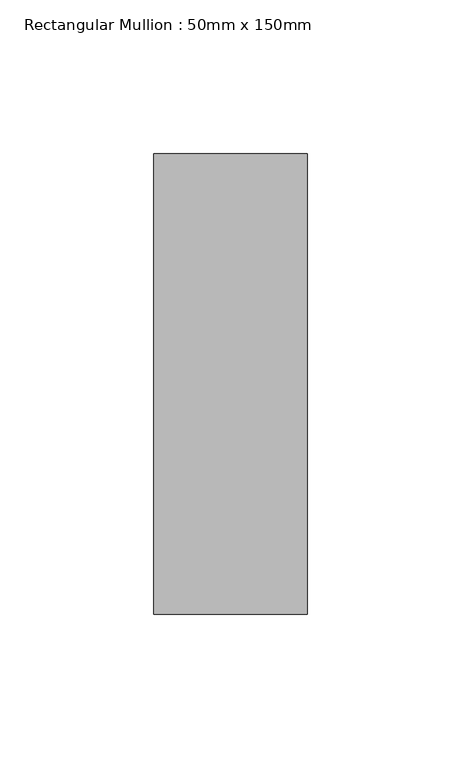
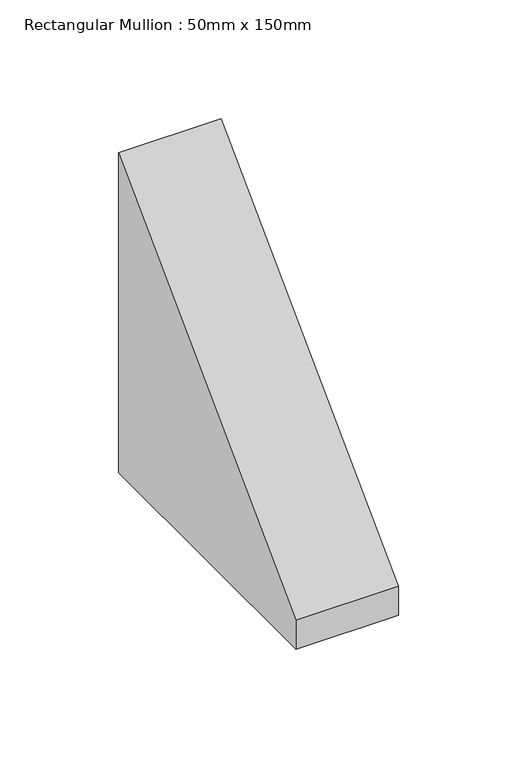
"""IFC4 building model written with IfcOpenShell, lengths in millimetres: member geometry, Rectangular Mullion : 50mm x 150mm."""

from ifc_helpers import new_model, si_unit, frame, origin, place, context, project, spatial, polyline, outline, extrude, source, transform, mapped, element, save


def rectangular_mullion_50mm_x_150mm_7b1b1d76(model_context):
    return source(origin(), model_context, "Body", "SweptSolid", [
        extrude(outline(polyline([(-75.0, -75.0), (75.0, 75.0), (75.0, -89.9999997), (-75.0, -89.9999997), (-75.0, -75.0)])), frame((-25.0, 0.0, 0.0), z_axis=(1.0, 0.0, 0.0), x_axis=(0.0, 1.0, 0.0)), (0.0, 0.0, 1.0), 50.0),
    ])


if __name__ == "__main__":
    model = new_model("IFC4")
    model_context = context("Model", 3, world=origin())
    ifc_project = project(units=[si_unit("LENGTHUNIT", "METRE", prefix="MILLI")], contexts=[model_context])
    site = spatial("IfcSite", under=ifc_project)
    building = spatial("IfcBuilding", under=site)
    placement = place(None, origin())
    rectangular_mullion_50mm_x_150mm_shape = rectangular_mullion_50mm_x_150mm_7b1b1d76(model_context)
    element("IfcMember", 1, ObjectType="Rectangular Mullion : 50mm x 150mm", at=placement, inside=building, context=model_context, shape_type="MappedRepresentation", body=[
        mapped(rectangular_mullion_50mm_x_150mm_shape, transform((0.0, 0.0, 0.0), x_axis=(1.0, 0.0, 0.0), y_axis=(0.0, 1.0, 0.0), z_axis=(0.0, 0.0, 1.0))),
    ])
    save(model, "model.ifc")

# Revit data of these elements
# Type "Rectangular Mullion : 50mm x 150mm"
#   built-in parameter 1007304 = 0.492126 (stored number, unit not read)
#   built-in parameter 1007301 = 0.082021 (stored number, unit not read)
#   built-in parameter 1007300 = 0.082021 (stored number, unit not read)
# Element 1 (IfcMember, "Rectangular Mullion : 50mm x 150mm")
#   Materials on its faces: "Aluminum"
# Materials
#   "Aluminum": class "Metal", colour RGB 244 244 244, transparency 0, Description = "Aluminum 6061", Cost = 0
